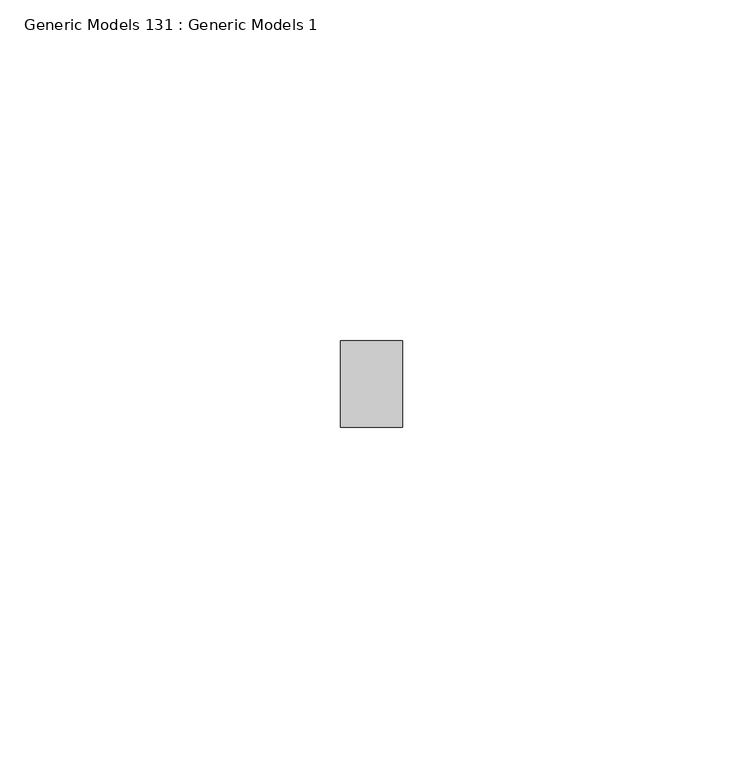
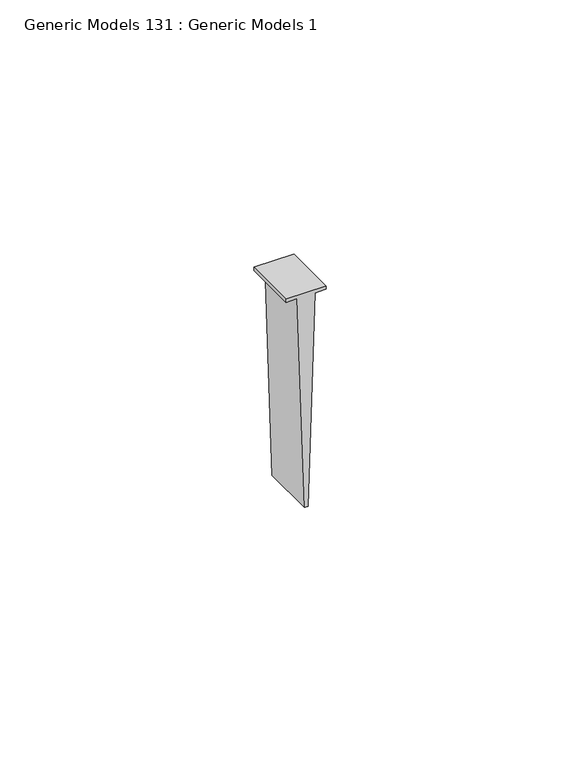
"""IFC4 building model written with IfcOpenShell, lengths in millimetres: proxy geometry, Generic Models 131 : Generic Models 1."""

from ifc_helpers import new_model, si_unit, frame, origin, place, context, project, spatial, polyline, outline, extrude, source, transform, mapped, element, save


def generic_models_131_generic_models_1_dfd9233a(model_context):
    return source(origin(), model_context, "Body", "SweptSolid", [
        extrude(outline(polyline([(-223.594817, 46885.2894531), (-224.388567, 46885.2894531), (-224.388567, 46887.8393167), (-275.188567, 46889.4367058), (-275.188567, 46890.2354003), (-224.388567, 46891.8327895), (-224.388567, 46894.3826531), (-223.594817, 46894.3826531), (-223.594817, 46885.2894531)])), frame((0.0, 565.15, 0.0), z_axis=(0.0, 1.0, 0.0), x_axis=(0.0, 0.0, 1.0)), (0.0, 0.0, 1.0), 12.7),
    ])


if __name__ == "__main__":
    model = new_model("IFC4")
    model_context = context("Model", 3, world=origin())
    ifc_project = project(units=[si_unit("LENGTHUNIT", "METRE", prefix="MILLI")], contexts=[model_context])
    site = spatial("IfcSite", under=ifc_project)
    building = spatial("IfcBuilding", under=site)
    placement = place(None, origin())
    generic_models_131_generic_models_1_shape = generic_models_131_generic_models_1_dfd9233a(model_context)
    element("IfcBuildingElementProxy", 1, Name="Generic Models 131 : Generic Models 1", ObjectType="Generic Models 131 : Generic Models 1", at=placement, inside=building, context=model_context, shape_type="MappedRepresentation", body=[
        mapped(generic_models_131_generic_models_1_shape, transform((0.0, 0.0, 0.0), x_axis=(1.0, 0.0, 0.0), y_axis=(0.0, 1.0, 0.0), z_axis=(0.0, 0.0, 1.0))),
    ])
    save(model, "model.ifc")

# Revit data of these elements
# Element 1 (IfcBuildingElementProxy, "Generic Models 131 : Generic Models 1")
#   Materials on its faces: "METAL RUNNER CHANNEL; FASTEN @ 24\" O.C."
# Materials
#   "METAL RUNNER CHANNEL; FASTEN @ 24\" O.C.": class "Unassigned", colour RGB 210 209 208, transparency 0, Keynote = "M05121300.02", Cost = 0
